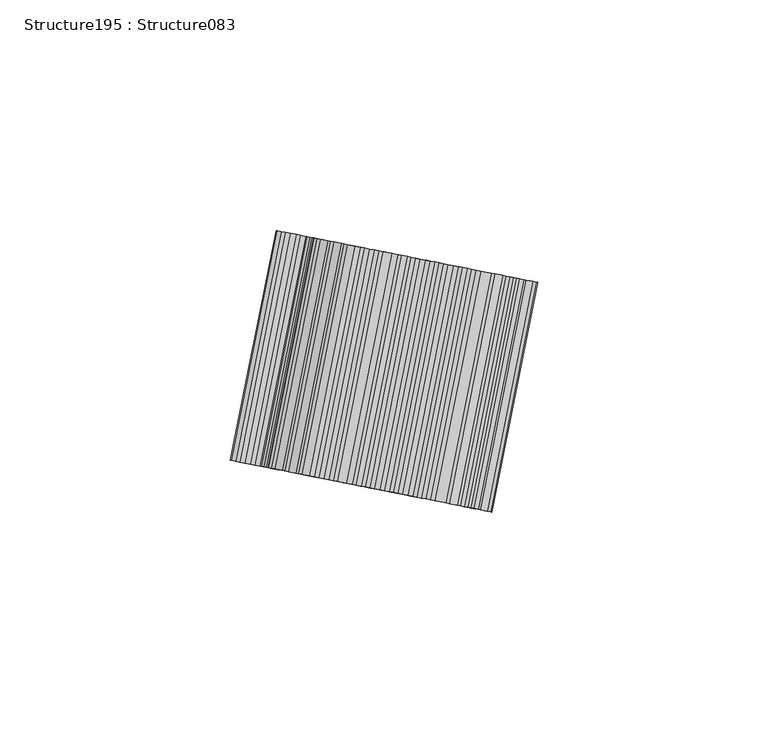
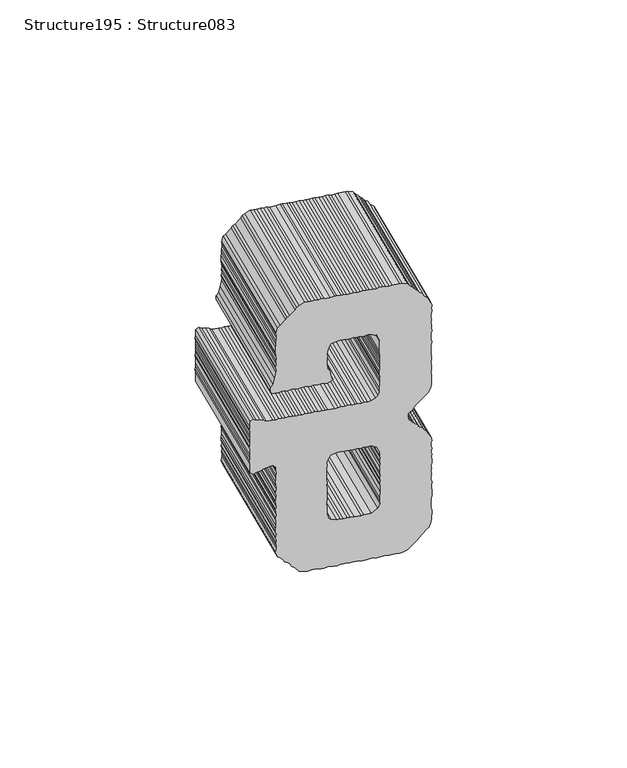
"""IFC4 building model written with IfcOpenShell, lengths in millimetres: proxy geometry, Structure195 : Structure083."""

from ifc_helpers import new_model, si_unit, frame, origin, place, context, project, spatial, polyline, outline, extrude, source, transform, mapped, element, save


def structure195_structure083_96396ef8(model_context):
    return source(origin(), model_context, "Body", "SweptSolid", [
        extrude(outline(polyline([(2.0811665, 0.0), (2.9845827, 0.2618804), (3.8993851, 0.1334309), (5.0653934, 0.1334309), (5.9801957, 0.0), (7.1465598, 0.1334309), (7.922594, 0.0), (9.0982094, 0.0), (10.2638618, 0.2618804), (11.3028439, 0.1334309), (12.3450283, 0.2618804), (13.3836546, 0.0), (15.072712, -0.7806598), (16.3682373, -2.3373539), (17.4104217, -2.7280396), (18.0572948, -3.7655983), (18.839022, -4.4131831), (19.362427, -5.0653934), (20.2676224, -5.8460532), (21.0529078, -6.7555183), (21.9570357, -7.4077286), (22.609246, -9.2263031), (22.4818639, -10.0023372), (22.4818639, -12.3446725), (22.3466539, -13.3825872), (22.3466539, -14.4205017), (22.609246, -15.3296111), (22.609246, -16.3675256), (22.3466539, -17.2816164), (22.3466539, -18.319531), (22.4818639, -19.6143446), (22.609246, -20.5284353), (22.4818639, -21.56635), (22.4818639, -22.4804406), (22.3466539, -23.5183553), (22.4818639, -24.55627), (22.3466539, -25.7272596), (22.3466539, -26.7651742), (22.4818639, -27.8030889), (22.4818639, -28.5837487), (22.609246, -29.8835437), (22.609246, -30.6642036), (22.3466539, -31.9639985), (22.3466539, -33.9110224), (22.609246, -34.8204876), (22.3466539, -35.8633836), (22.609246, -36.9009424), (22.4818639, -38.0673065), (22.4818639, -38.9767717), (22.609246, -40.1477613), (21.6940878, -41.8378863), (21.0529078, -42.6139205), (20.2676224, -43.1326999), (18.582123, -44.8228248), (18.0572948, -45.6038405), (17.4104217, -46.1226199), (15.5922031, -47.8127448), (14.9392811, -48.5934046), (13.1214183, -49.1125398), (12.2158672, -48.9840903), (11.3028439, -48.9840903), (10.1368356, -49.1125398), (8.9647784, -49.1125398), (7.922594, -49.2459707), (5.8474764, -49.2459707), (5.0653934, -49.1125398), (4.0267671, -48.9840903), (2.9845827, -49.1125398), (1.6911924, -48.9840903), (0.7817272, -49.2459707), (-0.3899741, -48.9840903), (-1.2990834, -49.1125398), (-3.246819, -49.6313192), (-5.3276296, -50.1500986), (-6.3644768, -50.8026647), (-7.5361781, -50.9261328), (-8.5790742, -50.411979), (-8.5790742, -49.6313192), (-8.7078795, -48.4599737), (-8.4456433, -47.2939654), (-8.4456433, -46.2510693), (-8.7078795, -45.3465857), (-8.4456433, -44.1755959), (-8.4456433, -43.2661308), (-8.7078795, -42.2282162), (-8.4456433, -40.1477613), (-8.4456433, -39.2386521), (-8.5790742, -38.195756), (-8.4456433, -37.0293919), (-8.7078795, -35.8633836), (-8.4456433, -34.9489371), (-8.4456433, -34.0398278), (-8.7078795, -33.0019131), (-8.4456433, -31.9639985), (-7.663916, -31.0499078), (-6.6270688, -31.7021181), (-4.2836661, -32.092448), (-3.5097668, -32.7400328), (-1.2990834, -33.0019131), (-0.3899741, -33.0019131), (1.0421844, -32.7400328), (1.8185744, -33.0019131), (2.9845827, -32.8684823), (4.8031571, -32.2208975), (5.4553675, -31.7021181), (5.8474764, -29.7501128), (6.1079336, -28.845629), (5.9801957, -27.6696579), (5.8474764, -26.5032939), (5.9801957, -25.7272596), (6.1079336, -24.422839), (5.9801957, -23.3849244), (6.1079336, -22.4804406), (5.8474764, -21.3044695), (6.1079336, -20.1381054), (6.1079336, -19.1001908), (5.0653934, -17.1481855), (2.9845827, -16.3675256), (-0.9091093, -16.3675256), (-2.2046346, -16.1106267), (-3.1176578, -16.1106267), (-4.1559283, -16.2390761), (-5.1988243, -16.2390761), (-6.2370947, -16.1106267), (-7.140511, -16.1106267), (-8.4456432, -16.3675256), (-9.3547526, -16.3675256), (-10.2642177, -16.2390761), (-11.435919, -16.2390761), (-12.3393353, -16.1106267), (-14.4205017, -16.3675256), (-15.7195851, -16.3675256), (-17.0243616, -16.7578556), (-17.6673207, -17.6673207), (-18.319531, -18.9717413), (-18.5824789, -20.1381054), (-18.319531, -21.17602), (-18.4529619, -22.0851294), (-18.319531, -23.3849244), (-18.4529619, -24.16594), (-18.5824789, -25.2034988), (-18.319531, -26.5032939), (-18.4529619, -27.2839536), (-18.319531, -28.4552992), (-18.4529619, -29.4932138), (-18.5824789, -30.6642036), (-18.5824789, -32.7400328), (-18.4529619, -33.649142), (-18.4529619, -34.5586072), (-18.5824789, -35.8633836), (-18.319531, -36.9009424), (-18.4529619, -37.8054261), (-18.4529619, -38.8479664), (-18.319531, -39.8858809), (-18.5824789, -41.0522451), (-18.4529619, -41.9663358), (-18.5824789, -42.8758009), (-18.319531, -43.9137155), (-18.319531, -45.0847053), (-18.4529619, -46.2510693), (-18.319531, -47.1651601), (-18.319531, -48.3315242), (-18.5824789, -49.2459707), (-18.319531, -50.2835295), (-18.319531, -52.2309093), (-17.6673207, -53.1400186), (-17.2773466, -54.4348322), (-17.1478297, -55.4777282), (-16.6286944, -56.3868376), (-17.2773466, -57.2963026), (-19.6186144, -57.2963026), (-20.4003417, -57.5532016), (-21.4371888, -57.4297335), (-22.736628, -57.2963026), (-23.6478722, -57.4297335), (-24.8174387, -57.2963026), (-25.5934729, -57.4297335), (-26.6360131, -57.5532016), (-27.6746394, -57.2963026), (-29.75545, -57.2963026), (-30.9214583, -57.4297335), (-31.8344816, -57.5532016), (-33.1300068, -57.2963026), (-36.1202826, -57.2963026), (-36.7724929, -56.3868376), (-36.2494437, -55.3489229), (-36.1202826, -54.3063827), (-35.5968776, -53.1400186), (-35.4677165, -52.1021039), (-34.8208434, -50.2835295), (-35.8576906, -49.1125398), (-36.899875, -49.1125398), (-37.9385012, -48.9840903), (-39.2379404, -49.1125398), (-40.1470497, -49.1125398), (-41.3187511, -49.2459707), (-43.1373255, -48.9840903), (-44.1759518, -48.9840903), (-45.3455182, -49.2459707), (-46.2567624, -48.9840903), (-47.1601787, -49.1125398), (-48.4653109, -49.2459707), (-49.3687272, -49.1125398), (-50.5404285, -48.9840903), (-51.3221558, -49.2459707), (-52.3590029, -49.1125398), (-53.5307043, -48.9840903), (-54.4398136, -49.2459707), (-55.6058219, -49.1125398), (-57.4243963, -49.1125398), (-58.4665807, -49.2459707), (-59.6386379, -49.2459707), (-60.6769083, -48.9840903), (-61.5863734, -49.2459707), (-62.6228648, -48.9840903), (-63.665405, -49.1125398), (-64.8331924, -48.9840903), (-65.7426575, -48.9840903), (-66.912224, -49.2459707), (-68.7268844, -48.5934046), (-69.2502894, -47.8127448), (-70.1593987, -46.9032797), (-71.068508, -46.3845002), (-71.7210742, -45.3465857), (-72.2345163, -44.6943753), (-73.2788356, -44.1755959), (-74.0587838, -43.1326999), (-75.6147662, -41.8378863), (-76.0065194, -40.0143304), (-76.1339014, -39.1102026), (-76.0065194, -37.938857), (-76.0065194, -36.1153012), (-76.2673323, -34.9489371), (-76.2673323, -33.9110224), (-76.0065194, -32.8684823), (-76.0065194, -31.9639985), (-76.2673323, -30.9264398), (-76.2673323, -29.6216633), (-76.0065194, -28.7121982), (-76.1339014, -27.6696579), (-76.0065194, -26.5032939), (-76.1339014, -25.7272596), (-76.0065194, -24.55627), (-76.0065194, -22.609246), (-76.2673323, -21.6947995), (-76.1339014, -20.3999858), (-76.0065194, -19.4858951), (-76.0065194, -18.4479805), (-76.2673323, -17.5434968), (-76.0065194, -15.463042), (-76.0065194, -14.1632469), (-76.2673323, -13.2491562), (-76.0065194, -12.0827921), (-76.0065194, -11.3021323), (-76.1339014, -10.0023372), (-76.0065194, -8.9644227), (-75.4873841, -7.4077286), (-74.8405111, -6.6270688), (-73.9257087, -5.7176037), (-72.4971084, -4.2893592), (-71.8502353, -3.7655983), (-70.8080509, -2.8564891), (-69.2502894, -1.2948136), (-68.7268844, -0.6522104), (-66.912224, 0.0), (-65.8700396, 0.1334309), (-64.7040313, 0.1334309), (-63.9240831, 0.2618804), (-62.7523817, 0.2618804), (-61.8468306, 0.0), (-58.4665807, 0.0), (-57.4243963, 0.2618804), (-55.4766608, 0.2618804), (-54.5671956, 0.1334309), (-53.6637794, 0.1334309), (-52.3590029, 0.2618804), (-51.3221558, 0.0), (-50.5404285, 0.0), (-49.3687272, 0.1334309), (-48.4653109, 0.0), (-47.1601787, 0.1334309), (-46.3841445, 0.0), (-45.3455182, 0.2618804), (-44.4324949, 0.2618804), (-43.1373255, 0.1334309), (-42.0947853, 0.2618804), (-41.185676, 0.0), (-40.0196677, 0.2618804), (-38.9771275, 0.0), (-37.9385012, 0.0), (-37.0293919, 0.2618804), (-35.8576906, 0.0), (-34.4290902, -0.7806598), (-33.5199809, -1.4282445), (-32.7400327, -2.2089044), (-31.8344816, -2.7280396), (-31.3114324, -3.7655983), (-30.4080162, -4.2893592), (-29.6223749, -5.3272738), (-28.8406477, -5.9794841), (-27.9372314, -6.7555183), (-27.1515902, -7.2742977), (-25.7229898, -7.2742977), (-24.5569815, -5.8460532), (-23.7752543, -5.3272738), (-22.866145, -4.546614), (-21.4371888, -2.9849386), (-20.5241656, -2.0804549), (-19.2286403, -0.7806598), (-17.5378038, 0.0), (-16.3717955, 0.1334309), (-13.2541376, 0.1334309), (-12.2119532, 0.0), (-11.435919, 0.1334309), (-10.1347007, 0.1334309), (-8.4456433, 0.0), (-7.4034588, 0.1334309), (-6.2370947, 0.1334309), (-5.3276296, 0.0), (-2.2046346, 0.0), (-1.0386263, 0.2618804), (0.0, 0.0), (2.0811665, 0.0)]), holes=[polyline([(-35.4677165, -31.7021181), (-34.8208434, -29.8835437), (-34.8208434, -28.7121982), (-34.9482254, -27.9315384), (-34.8208434, -26.6317434), (-34.9482254, -25.4653792), (-35.0816564, -24.55627), (-34.8208434, -23.5183553), (-35.0816564, -22.4804406), (-34.8208434, -21.17602), (-34.9482254, -20.3999858), (-34.8208434, -19.1001908), (-35.7303085, -17.2816164), (-37.6759092, -16.3675256), (-38.9771275, -16.3675256), (-39.8865926, -16.2390761), (-40.9230839, -16.3675256), (-42.0947853, -16.1106267), (-43.1373255, -16.3675256), (-45.0850611, -16.3675256), (-46.1215524, -16.2390761), (-47.2936096, -16.3675256), (-48.2027189, -16.1106267), (-49.3687272, -16.3675256), (-50.1543684, -16.1106267), (-52.3590029, -16.1106267), (-54.4398136, -16.3675256), (-55.6058219, -16.3675256), (-56.6483621, -16.2390761), (-58.2061236, -17.019736), (-59.505207, -19.1001908), (-59.505207, -21.4379005), (-59.6386379, -22.2185603), (-59.6386379, -24.422839), (-59.3760458, -25.7272596), (-59.505207, -26.6317434), (-59.505207, -27.9315384), (-59.3760458, -28.845629), (-59.505207, -29.8835437), (-58.8529967, -31.7021181), (-58.3391987, -32.3543285), (-56.5209801, -32.7400328), (-55.4766608, -32.8684823), (-54.3067385, -32.8684823), (-53.2681123, -33.0019131), (-52.2316209, -33.0019131), (-51.4495378, -32.8684823), (-50.4073534, -32.7400328), (-49.2413451, -32.8684823), (-47.2936096, -32.8684823), (-45.9941704, -33.0019131), (-45.2181362, -32.7400328), (-43.9133597, -33.0019131), (-40.0196677, -33.0019131), (-38.8479663, -32.7400328), (-37.6759092, -33.0019131), (-36.2494437, -32.2208975), (-35.4677165, -31.7021181)])]), frame((-2844.3041246, 235032.9546988, 462.795938), z_axis=(0.19466222296394123, 0.9808703374813295, 0.0), x_axis=(0.0, 0.0, 1.0)), (0.0, 0.0, 1.0), 50.8),
    ])


if __name__ == "__main__":
    model = new_model("IFC4")
    model_context = context("Model", 3, world=origin())
    ifc_project = project(units=[si_unit("LENGTHUNIT", "METRE", prefix="MILLI")], contexts=[model_context])
    site = spatial("IfcSite", under=ifc_project)
    building = spatial("IfcBuilding", under=site)
    placement = place(None, origin())
    structure195_structure083_shape = structure195_structure083_96396ef8(model_context)
    element("IfcBuildingElementProxy", 1, Name="Structure195 : Structure083", ObjectType="Structure195 : Structure083", at=placement, inside=building, context=model_context, shape_type="MappedRepresentation", body=[
        mapped(structure195_structure083_shape, transform((0.0, 0.0, 0.0), x_axis=(1.0, 0.0, 0.0), y_axis=(0.0, 1.0, 0.0), z_axis=(0.0, 0.0, 1.0))),
    ])
    save(model, "model.ifc")

# Revit data of these elements
# Type "Structure195 : Structure083"
#   NameOverride = "Structure083"
# Element 1 (IfcBuildingElementProxy, "Structure195 : Structure083")
#   Materials on its faces: "BRUSHED ALUMINUM LETTERING"
# Materials
#   "BRUSHED ALUMINUM LETTERING": class "Unassigned", colour RGB 169 181 186, transparency 0, Cost = 0
